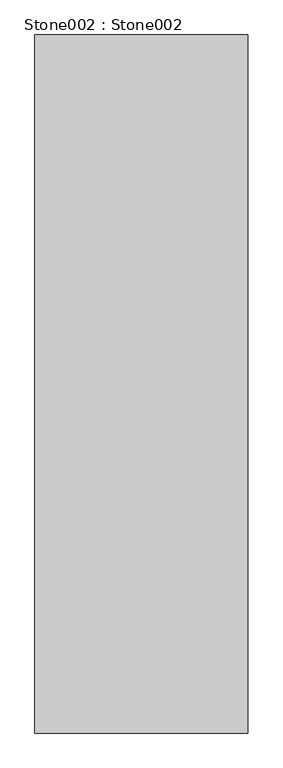
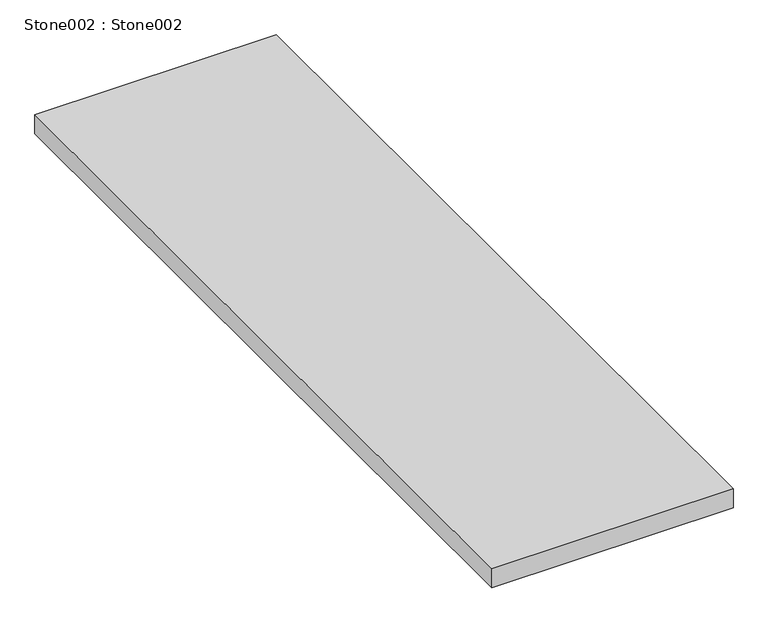
"""IFC4 building model written with IfcOpenShell, lengths in millimetres: proxy geometry, Stone002 : Stone002."""

from ifc_helpers import new_model, si_unit, frame, origin, place, context, project, spatial, polyline, outline, extrude, source, transform, mapped, element, save


def stone002_stone002_c6ba8601(model_context):
    return source(origin(), model_context, "Body", "SweptSolid", [
        extrude(outline(polyline([(-4250.4517696, -1052.8906574), (-4860.0517696, -1052.8906574), (-4860.0517696, 947.1093426), (-4250.4517696, 947.1093426), (-4250.4517696, -1052.8906574)])), frame((0.0, 0.0, 36508.2444375), z_axis=(0.0, 0.0, 1.0), x_axis=(1.0, 0.0, 0.0)), (0.0, 0.0, 1.0), 50.8),
    ])


if __name__ == "__main__":
    model = new_model("IFC4")
    model_context = context("Model", 3, world=origin())
    ifc_project = project(units=[si_unit("LENGTHUNIT", "METRE", prefix="MILLI")], contexts=[model_context])
    site = spatial("IfcSite", under=ifc_project)
    building = spatial("IfcBuilding", under=site)
    placement = place(None, origin())
    stone002_stone002_shape = stone002_stone002_c6ba8601(model_context)
    element("IfcBuildingElementProxy", 1, Name="Stone002 : Stone002", ObjectType="Stone002 : Stone002", at=placement, inside=building, context=model_context, shape_type="MappedRepresentation", body=[
        mapped(stone002_stone002_shape, transform((0.0, 0.0, 0.0), x_axis=(1.0, 0.0, 0.0), y_axis=(0.0, 1.0, 0.0), z_axis=(0.0, 0.0, 1.0))),
    ])
    save(model, "model.ifc")

# Revit data of these elements
# Type "Stone002 : Stone002"
#   NameOverride = "Stone002"
# Element 1 (IfcBuildingElementProxy, "Stone002 : Stone002")
#   Materials on its faces: "2\" STONE DECK TBD"
# Materials
#   "2\" STONE DECK TBD": class "Unassigned", colour RGB 199 185 173, transparency 0
